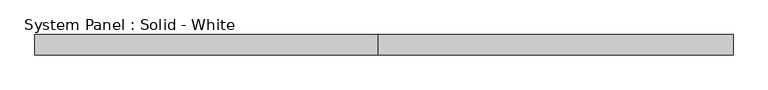
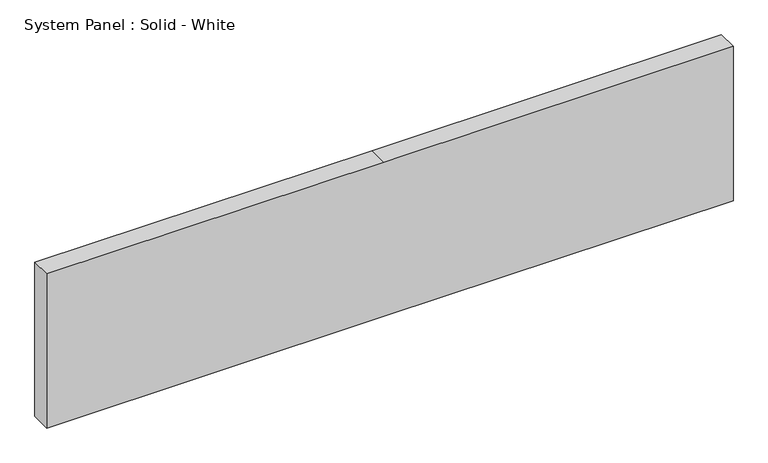
"""IFC4 building model written with IfcOpenShell, lengths in millimetres: plate geometry, System Panel : Solid - White."""

from ifc_helpers import new_model, si_unit, frame, origin, place, context, project, spatial, polyline, outline, extrude, source, transform, mapped, element, save


def system_panel_solid_white_afab91cb(model_context):
    return source(origin(), model_context, "Body", "SweptSolid", [
        extrude(outline(polyline([(0.0, -1082.8418644), (0.0, -18.5818644), (0.0, 1082.8418644), (514.35, 1082.8418644), (514.35, -18.5818644), (514.35, -1082.8418644), (0.0, -1082.8418644)])), frame((0.0, -19.05, 0.0), z_axis=(0.0, 1.0, 0.0), x_axis=(0.0, 0.0, 1.0)), (0.0, 0.0, 1.0), 63.5),
    ])


if __name__ == "__main__":
    model = new_model("IFC4")
    model_context = context("Model", 3, world=origin())
    ifc_project = project(units=[si_unit("LENGTHUNIT", "METRE", prefix="MILLI")], contexts=[model_context])
    site = spatial("IfcSite", under=ifc_project)
    building = spatial("IfcBuilding", under=site)
    placement = place(None, origin())
    system_panel_solid_white_shape = system_panel_solid_white_afab91cb(model_context)
    element("IfcPlate", 1, ObjectType="System Panel : Solid - White", at=placement, inside=building, context=model_context, shape_type="MappedRepresentation", body=[
        mapped(system_panel_solid_white_shape, transform((0.0, 0.0, 0.0), x_axis=(1.0, 0.0, 0.0), y_axis=(0.0, 1.0, 0.0), z_axis=(0.0, 0.0, 1.0))),
    ])
    save(model, "model.ifc")

# Revit data of these elements
# Element 1 (IfcPlate, "System Panel : Solid - White")
#   Materials on its faces: "White Panel"
# Materials
#   "White Panel": class "Unassigned", colour RGB 255 255 255, transparency 0
